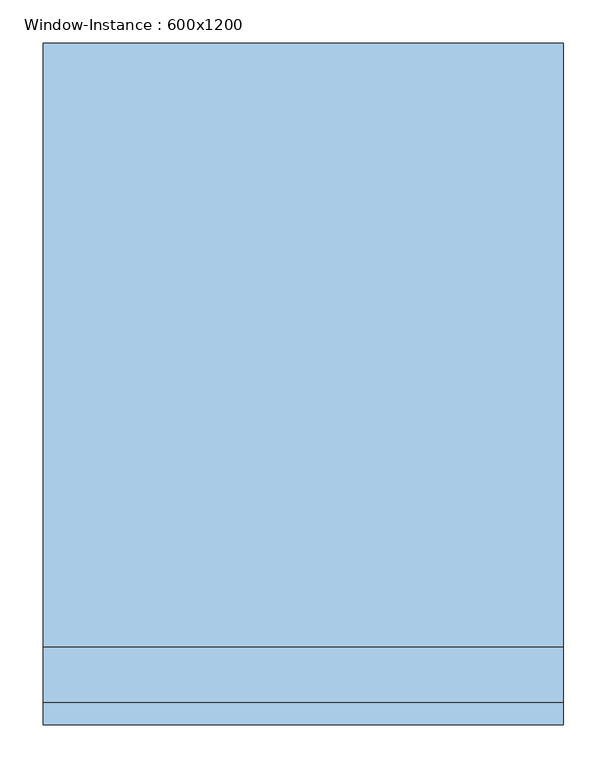
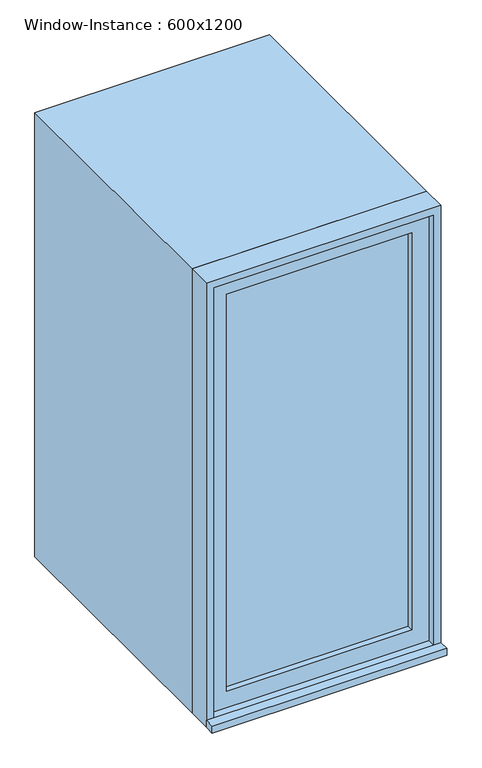
"""IFC4 building model written with IfcOpenShell, lengths in millimetres: window geometry, Window-Instance : 600x1200."""

import ifcopenshell
import ifcopenshell.guid

model = None  # the IFC model being written
_history = None  # IfcOwnerHistory: only IFC2X3 demands one
_inside = {}  # id of a spatial element -> (the spatial element, [elements in it])
_under = {}  # id of a project, library or spatial element -> (it, [spatial elements below it])
_declared = {}  # id of a project -> (the project, [libraries it declares])
_typed = {}  # id of a type object -> (the type object, [elements of that type])
_made_of = {}  # id of a material, layer set ... -> (it, [elements and type objects made of it])


def new_model(schema):
    """Start an empty IFC model of exactly this schema.

    Asked for "IFC4X3", IfcOpenShell would pick the latest addendum, in which some entities
    have other attributes; the version numbers below select the first issue.
    IFC2X3 requires an IfcOwnerHistory on every rooted entity: one is made here for all.
    """
    global model, _history
    if schema == "IFC4X3":
        model = ifcopenshell.file(schema_version=(4, 3, 0, 0))
    else:
        model = ifcopenshell.file(schema=schema)
    _inside.clear()
    _under.clear()
    _declared.clear()
    _typed.clear()
    _made_of.clear()
    _history = None
    if model.schema == "IFC2X3":
        org = make("IfcOrganization", Name="unknown")
        user = make(
            "IfcPersonAndOrganization",
            ThePerson=make("IfcPerson", FamilyName="unknown"),
            TheOrganization=org,
        )
        app = make(
            "IfcApplication",
            ApplicationDeveloper=org,
            Version="unknown",
            ApplicationFullName="unknown",
            ApplicationIdentifier="unknown",
        )
        _history = make(
            "IfcOwnerHistory",
            OwningUser=user,
            OwningApplication=app,
            ChangeAction="ADDED",
            CreationDate=0,
        )
    return model


def make(cls, **values):
    """One entity of the class cls with the attributes given. An attribute that is None is left unset."""
    return model.create_entity(
        cls, **{name: value for name, value in values.items() if value is not None}
    )


def rooted(cls, **values):
    """An entity with a GlobalId (a new one), such as an element, a storey or a relation."""
    return make(cls, GlobalId=ifcopenshell.guid.new(), OwnerHistory=_history, **values)


def si_unit(unit_type, name, prefix=None):
    """IfcSIUnit, for example si_unit("LENGTHUNIT", "METRE", prefix="MILLI")."""
    return make("IfcSIUnit", UnitType=unit_type, Prefix=prefix, Name=name)


def assignment(units):
    """IfcUnitAssignment: the units of a project."""
    return None if units is None else make("IfcUnitAssignment", Units=units)


def point(xyz):
    """IfcCartesianPoint."""
    return None if xyz is None else make("IfcCartesianPoint", Coordinates=xyz)


def direction(xyz):
    """IfcDirection."""
    return None if xyz is None else make("IfcDirection", DirectionRatios=xyz)


def frame(location, z_axis=None, x_axis=None):
    """IfcAxis2Placement3D, a coordinate frame: its origin and axes. An axis left out is left unset."""
    return make(
        "IfcAxis2Placement3D",
        Location=point(location),
        Axis=direction(z_axis),
        RefDirection=direction(x_axis),
    )


def origin():
    """The frame at (0, 0, 0) with its axes left unset."""
    return frame((0.0, 0.0, 0.0))


def place(relative_to, where):
    """IfcLocalPlacement: puts the frame where relative to a parent placement (None: the world)."""
    return make(
        "IfcLocalPlacement", PlacementRelTo=relative_to, RelativePlacement=where
    )


def context(
    kind, dimensions, precision=None, world=None, true_north=None, identifier=None
):
    """IfcGeometricRepresentationContext, for example the 3D "Model" context."""
    return make(
        "IfcGeometricRepresentationContext",
        ContextIdentifier=identifier,
        ContextType=kind,
        CoordinateSpaceDimension=dimensions,
        Precision=precision,
        WorldCoordinateSystem=world,
        TrueNorth=true_north,
    )


def project(units=None, contexts=None):
    """IfcProject with its units and contexts."""
    return rooted(
        "IfcProject",
        Name="project",
        RepresentationContexts=contexts,
        UnitsInContext=assignment(units),
    )


def spatial(cls, under=None, at=None, **own):
    """A site, building, storey or space (cls), placed at a placement, below another one or the project."""
    s = rooted(cls, ObjectPlacement=at, **own)
    if under is not None:
        _under.setdefault(under.id(), (under, []))[1].append(s)
    return s


def polyline(points):
    """IfcPolyline through the points."""
    return make("IfcPolyline", Points=[point(p) for p in points])


def outline(outer, holes=None, kind="AREA"):
    """IfcArbitraryClosedProfileDef: a profile drawn as a closed curve; with holes, ...WithVoids."""
    if holes is None:
        return make("IfcArbitraryClosedProfileDef", ProfileType=kind, OuterCurve=outer)
    return make(
        "IfcArbitraryProfileDefWithVoids",
        ProfileType=kind,
        OuterCurve=outer,
        InnerCurves=holes,
    )


def extrude(swept, where, along, depth):
    """IfcExtrudedAreaSolid: the profile swept, set in the frame where, extruded along a direction by depth."""
    return make(
        "IfcExtrudedAreaSolid",
        SweptArea=swept,
        Position=where,
        ExtrudedDirection=direction(along),
        Depth=depth,
    )


def shape(context_of_items, identifier, shape_type, items):
    """IfcShapeRepresentation: the items that make up one representation, for example the "Body"."""
    return make(
        "IfcShapeRepresentation",
        ContextOfItems=context_of_items,
        RepresentationIdentifier=identifier,
        RepresentationType=shape_type,
        Items=items,
    )


def source(mapping_origin, context_of_items, identifier, shape_type, items):
    """IfcRepresentationMap: a shape defined once, which mapped items show again and again."""
    return make(
        "IfcRepresentationMap",
        MappingOrigin=mapping_origin,
        MappedRepresentation=shape(context_of_items, identifier, shape_type, items),
    )


def transform(
    local_origin,
    x_axis=None,
    y_axis=None,
    z_axis=None,
    scale=None,
    scale2=None,
    scale3=None,
    uniform=True,
):
    """IfcCartesianTransformationOperator3D, or its non-uniform kind. x_axis, y_axis, z_axis: its Axis1, 2, 3."""
    if uniform:
        return make(
            "IfcCartesianTransformationOperator3D",
            Axis1=direction(x_axis),
            Axis2=direction(y_axis),
            LocalOrigin=point(local_origin),
            Scale=scale,
            Axis3=direction(z_axis),
        )
    return make(
        "IfcCartesianTransformationOperator3DnonUniform",
        Axis1=direction(x_axis),
        Axis2=direction(y_axis),
        LocalOrigin=point(local_origin),
        Scale=scale,
        Axis3=direction(z_axis),
        Scale2=scale2,
        Scale3=scale3,
    )


def mapped(mapping_source, mapping_target):
    """IfcMappedItem: shows the shape of a source again, moved by a transform."""
    return make(
        "IfcMappedItem", MappingSource=mapping_source, MappingTarget=mapping_target
    )


def made_of(thing, what):
    """Note that an element or type object is made of a material, layer set ...; save() writes the relation."""
    if what is not None:
        _made_of.setdefault(what.id(), (what, []))[1].append(thing)
    return thing


def element(
    cls,
    number,
    at=None,
    inside=None,
    cuts=None,
    type_object=None,
    material=None,
    context=None,
    identifier="Body",
    shape_type=None,
    held_by="IfcProductDefinitionShape",
    body=None,
    shapes=None,
    **own,
):
    """One element of the class cls, such as IfcWall. Its Tag is "e" and its number.

    at: its placement. inside: the storey or other place that contains it. cuts: it is an
    opening in that element (IfcRelVoidsElement). A single representation is given by context,
    identifier, shape_type and body (its items); several are given by shapes. held_by: the class
    of the entity that holds the representations. save() writes the other relations.
    """
    e = rooted(cls, Tag="e%d" % number, ObjectPlacement=at, **own)
    if body is not None:
        shapes = [shape(context, identifier, shape_type, body)]
    if shapes is not None:
        e.Representation = make(held_by, Representations=shapes)
    if inside is not None:
        _inside.setdefault(inside.id(), (inside, []))[1].append(e)
    if cuts is not None:
        rooted(
            "IfcRelVoidsElement", RelatingBuildingElement=cuts, RelatedOpeningElement=e
        )
    if type_object is not None:
        _typed.setdefault(type_object.id(), (type_object, []))[1].append(e)
    return made_of(e, material)


def aggregate(whole, parts):
    """IfcRelAggregates: a whole, such as a stair, and the parts it consists of."""
    return rooted("IfcRelAggregates", RelatingObject=whole, RelatedObjects=parts)


def save(model, path):
    """Write the relations noted so far, then the file.

    IfcRelAggregates (storeys below a building ...), IfcRelContainedInSpatialStructure (elements
    in a storey), IfcRelDefinesByType, IfcRelAssociatesMaterial and IfcRelDeclares: one each for
    every whole, place, type object, material and project.
    """
    for whole, parts in _under.values():
        aggregate(whole, parts)
    for where, things in _inside.values():
        rooted(
            "IfcRelContainedInSpatialStructure",
            RelatedElements=things,
            RelatingStructure=where,
        )
    for kind, things in _typed.values():
        rooted("IfcRelDefinesByType", RelatedObjects=things, RelatingType=kind)
    for what, things in _made_of.values():
        rooted("IfcRelAssociatesMaterial", RelatedObjects=things, RelatingMaterial=what)
    for by, libraries in _declared.values():
        rooted("IfcRelDeclares", RelatingContext=by, RelatedDefinitions=libraries)
    model.write(path)


def window_instance_600x1200_935e6ff8(model_context):
    return source(origin(), model_context, "Body", "SweptSolid", [
        extrude(outline(polyline([(-338.1, -405.4), (-338.1, -380.0), (261.9, -380.0), (261.9, -405.4), (-338.1, -405.4)])), frame((0.0, 0.0, 900.0), z_axis=(0.0, 0.0, 1.0), x_axis=(1.0, 0.0, 0.0)), (0.0, 0.0, 1.0), 19.05),
        extrude(outline(polyline([(198.4, -331.425), (198.4, -344.125), (-274.6, -344.125), (-274.6, -331.425), (198.4, -331.425)])), frame((0.0, 0.0, 963.5), z_axis=(0.0, 0.0, 1.0), x_axis=(1.0, 0.0, 0.0)), (0.0, 0.0, 1.0), 1073.0),
        extrude(outline(polyline([(2080.95, -319.05), (919.05, -319.05), (919.05, 242.85), (2080.95, 242.85), (2080.95, -319.05)]), holes=[polyline([(2036.5, -274.6), (2036.5, 198.4), (963.5, 198.4), (963.5, -274.6), (2036.5, -274.6)])]), frame((0.0, -360.0, 0.0), z_axis=(0.0, 1.0, 0.0), x_axis=(0.0, 0.0, 1.0)), (0.0, 0.0, 1.0), 44.45),
        extrude(outline(polyline([(2100.0, -338.1), (900.0, -338.1), (900.0, 261.9), (2100.0, 261.9), (2100.0, -338.1)]), holes=[polyline([(2068.25, -306.35), (2068.25, 230.15), (931.75, 230.15), (931.75, -306.35), (2068.25, -306.35)])]), frame((0.0, -315.55, 0.0), z_axis=(0.0, 1.0, 0.0), x_axis=(0.0, 0.0, 1.0)), (0.0, 0.0, 1.0), 695.55),
        extrude(outline(polyline([(2100.0, 261.9), (2100.0, -338.1), (900.0, -338.1), (900.0, 261.9), (2100.0, 261.9)]), holes=[polyline([(2080.95, 242.85), (919.05, 242.85), (919.05, -319.05), (2080.95, -319.05), (2080.95, 242.85)])]), frame((0.0, -380.0, 0.0), z_axis=(0.0, 1.0, 0.0), x_axis=(0.0, 0.0, 1.0)), (0.0, 0.0, 1.0), 64.45),
    ])


if __name__ == "__main__":
    model = new_model("IFC4")
    model_context = context("Model", 3, world=origin())
    ifc_project = project(units=[si_unit("LENGTHUNIT", "METRE", prefix="MILLI")], contexts=[model_context])
    site = spatial("IfcSite", under=ifc_project)
    building = spatial("IfcBuilding", under=site)
    placement = place(None, origin())
    window_instance_600x1200_shape = window_instance_600x1200_935e6ff8(model_context)
    element("IfcWindow", 1, ObjectType="Window-Instance : 600x1200", at=placement, inside=building, context=model_context, shape_type="MappedRepresentation", body=[
        mapped(window_instance_600x1200_shape, transform((0.0, 0.0, 0.0), x_axis=(1.0, 0.0, 0.0), y_axis=(0.0, 1.0, 0.0), z_axis=(0.0, 0.0, 1.0))),
    ])
    save(model, "model.ifc")

# Revit data of these elements
# Type "Window-Instance : 600x1200"
#   Type Mark = "7"
#   Construction Type Id = "GSP4R"
#   Assembly Code = "B2020100"
#   Analytic Construction = "1/8 in Pilkington single glazing"
#   Visual Light Transmittance = 0.9
#   Thermal Resistance (R) = 0.149095 (m²·K)/W
#   Solar Heat Gain Coefficient = 0.86
#   Heat Transfer Coefficient (U) = 6.70716 W/(m²·K)
#   Height [instance default] = 1200 mm
#   Default Sill Height = 900 mm
#   Width [instance default] = 600 mm
#   Window Inset = 20 mm
#   Glass Pane Material = WW-EC-GL-Storefront
#   Sash Material = WW-EC-RGB-White
#   Wall Closure = (empty or 0)
# Element 1 (IfcWindow, "Window-Instance : 600x1200")
#   Materials on its faces: "WW-EC-RGB-White", "WW-EC-GL-Storefront"
# Materials
#   "WW-EC-GL-Storefront": class "Glass", colour RGB 236 240 239, transparency 0.85, Description = "Storefront Glass", Cost = 0
#   "WW-EC-RGB-White": class "Generic", colour RGB 255 255 255, transparency 0, Comments = "If region requests off-white, swith asset color to RGB 231-228-220", Description = "Generic Color", Cost = 0
